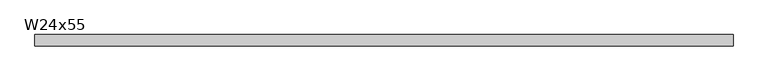
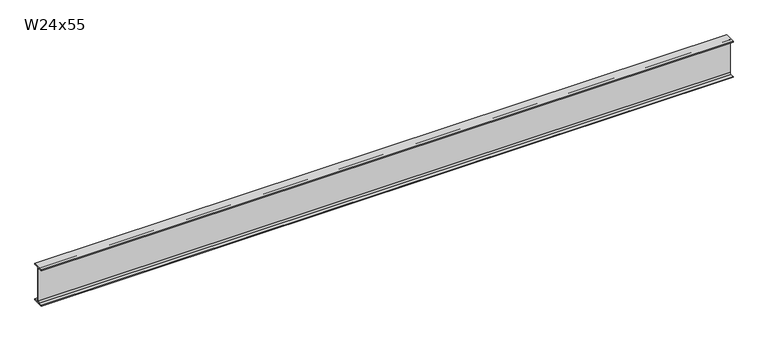
"""IFC4 building model written with IfcOpenShell, lengths in millimetres: beam geometry, RME W-Wide Flange : W24x55."""

from ifc_helpers import new_model, si_unit, point, frame, frame_2d, origin, place, context, project, spatial, polyline, circle_curve, trimmed, segment, composite_curve, outline, extrude, source, transform, mapped, element, save


def w24x55_0fa592e8(model_context):
    return source(origin(), model_context, "Body", "SweptSolid", [
        extrude(outline(composite_curve([segment(polyline([(89.027, -286.893), (89.027, -299.72), (-89.027, -299.72), (-89.027, -286.893), (-28.702, -286.893)]), True, "CONTINUOUS"), segment(trimmed(circle_curve(frame_2d((-28.702, -263.2075)), 23.6855), [point((-28.702, -286.893))], [point((-5.0165, -263.2075))], True, "CARTESIAN"), True, "CONTINUOUS"), segment(polyline([(-5.0165, -263.2075), (-5.0165, 263.2075)]), True, "CONTINUOUS"), segment(trimmed(circle_curve(frame_2d((-28.702, 263.2075)), 23.6855), [point((-5.0165, 263.2075))], [point((-28.702, 286.893))], True, "CARTESIAN"), True, "CONTINUOUS"), segment(polyline([(-28.702, 286.893), (-89.027, 286.893), (-89.027, 299.72), (89.027, 299.72), (89.027, 286.893), (28.702, 286.893)]), True, "CONTINUOUS"), segment(trimmed(circle_curve(frame_2d((28.702, 263.2075)), 23.6855), [point((28.702, 286.893))], [point((5.0165, 263.2075))], True, "CARTESIAN"), True, "CONTINUOUS"), segment(polyline([(5.0165, 263.2075), (5.0165, -263.2075)]), True, "CONTINUOUS"), segment(trimmed(circle_curve(frame_2d((28.702, -263.2075)), 23.6855), [point((5.0165, -263.2075))], [point((28.702, -286.893))], True, "CARTESIAN"), True, "CONTINUOUS"), segment(polyline([(28.702, -286.893), (89.027, -286.893)]), True, "CONTINUOUS")], self_intersect=False)), frame((-5377.8937141, 0.0, 0.0), z_axis=(1.0, 0.0, 0.0), x_axis=(0.0, 1.0, 0.0)), (0.0, 0.0, 1.0), 10869.1984283),
    ])


if __name__ == "__main__":
    model = new_model("IFC4")
    model_context = context("Model", 3, world=origin())
    ifc_project = project(units=[si_unit("LENGTHUNIT", "METRE", prefix="MILLI")], contexts=[model_context])
    site = spatial("IfcSite", under=ifc_project)
    building = spatial("IfcBuilding", under=site)
    placement = place(None, origin())
    w24x55_shape = w24x55_0fa592e8(model_context)
    element("IfcBeam", 1, ObjectType="RME W-Wide Flange : W24x55", at=placement, inside=building, context=model_context, shape_type="MappedRepresentation", body=[
        mapped(w24x55_shape, transform((0.0, 0.0, 0.0), x_axis=(1.0, 0.0, 0.0), y_axis=(0.0, 1.0, 0.0), z_axis=(0.0, 0.0, 1.0))),
    ])
    save(model, "model.ifc")

# Revit data of these elements
# Type "RME W-Wide Flange : W24x55"
#   WELD P [instance default] = ""
#   WELD LE [instance default] = ""
#   WELD D [instance default] = ""
#   TOP SECTION SIZE [instance default] = ""
#   TOP SECTION LENGTH [instance default] = ""
#   REMARKS [instance default] = ""
#   REINF TYPE [instance default] = ""
#   Nominal Size = "W24"
#   End Bearing Capacity [instance default] = ""
#   BOT SECTION SIZE [instance default] = ""
#   BOT SECTION LENGTH [instance default] = ""
#   Assembly Code = "B10"
#   W = 55
#   Start Extension Calculation [instance default] = 10' - 0"
#   Start Extension [instance default] = -0' - 0 1/2"
#   End Extension Calculation [instance default] = 10' - 0"
#   End Extension [instance default] = -0' - 0 1/2"
#   Length [instance default] = 5' - 0"
#   bf = 0' - 7.01"
#   d = 1' - 11.6"
#   k = 0' - 1 7/16"
#   k2 = 0' - 0.9325"
#   tf = 0' - 0.505"
#   tw = 0' - 0.395"
#   A = 0.1125 SF
#   Structural Material [instance default] = Metal - Steel - ASTM A992
# Element 1 (IfcBeam, "RME W-Wide Flange : W24x55")
#   Length = 36' - 0.3862"
#   Materials on its faces: "Metal - Steel - ASTM A992"
# Materials
#   "Metal - Steel - ASTM A992": class "Metal", colour RGB 255 128 0, transparency 0
